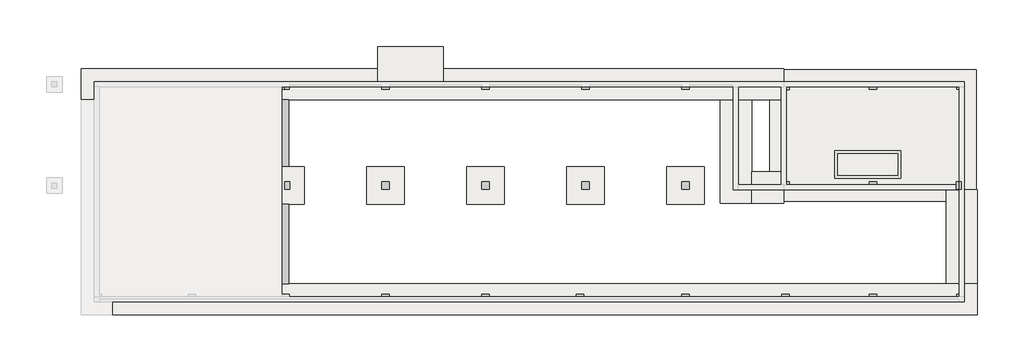
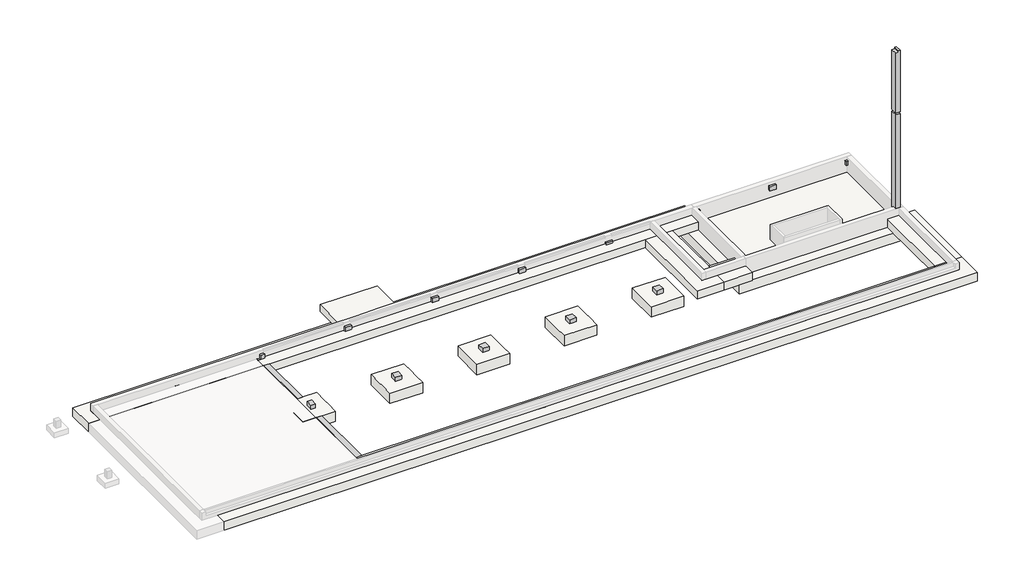
# Not in any storey, part 2 of 2: 25 columns, 8 beams, 8 slabs, 5 footings.
"""IFC4 building model written with IfcOpenShell, lengths in millimetres."""

from ifc_helpers import new_model, si_unit, frame, origin, place, context, project, spatial, polyline, outline, extrude, faceted_brep, element, save

model = new_model("IFC4")

# Units and contexts
model_context = context("Model", 3, world=origin())
ifc_project = project(units=[si_unit("LENGTHUNIT", "METRE", prefix="MILLI")], contexts=[model_context])

# Site, building
site = spatial("IfcSite", under=ifc_project)
building = spatial("IfcBuilding", under=site)

# Beams
placement = place(None, origin())
element("IfcBeam", 1, ObjectType="RC Beam_Rectangular : H_SB_AR_S16_FG_B600xH800_FG2", at=placement, inside=building, context=model_context, shape_type="Brep", body=[
    faceted_brep([(1150.0, 9199.5208589, -1350.0381366), (6000.0, 9199.5208589, -1350.0381366), (6000.0, 9199.5208589, -700.0381366), (4000.0, 9199.5208589, -700.0381366), (3500.0, 9199.5208589, -700.0381366), (1150.0, 9199.5208589, -700.0381366), (1150.0, 9799.5208589, -1350.0381366), (6000.0, 9799.5208589, -1350.0381366), (1150.0, 9799.5208589, -700.0381366), (3500.0, 9799.5208589, -700.0381366), (4000.0, 9799.5208589, -700.0381366), (6000.0, 9799.5208589, -700.0381366)], [[[0, 1, 2, 3, 4, 5]], [[0, 6, 7, 1]], [[7, 6, 8, 9, 10, 11]], [[6, 0, 5, 8]], [[1, 7, 11, 2]], [[5, 4, 3, 2, 11, 10, 9, 8]]]),
])
element("IfcBeam", 2, ObjectType="RC Beam_Rectangular : H_SB_AR_S16_FG_B600xH800_FG2", at=placement, inside=building, context=model_context, shape_type="Brep", body=[
    faceted_brep([(9000.0, 9199.5208589, -1350.0381366), (13500.0, 9199.5208589, -1350.0381366), (13500.0, 9199.5208589, -700.0381366), (11500.0, 9199.5208589, -700.0381366), (11000.0, 9199.5208589, -700.0381366), (9000.0, 9199.5208589, -700.0381366), (9000.0, 9799.5208589, -1350.0381366), (13500.0, 9799.5208589, -1350.0381366), (9000.0, 9799.5208589, -700.0381366), (11000.0, 9799.5208589, -700.0381366), (11500.0, 9799.5208589, -700.0381366), (13500.0, 9799.5208589, -700.0381366)], [[[0, 1, 2, 3, 4, 5]], [[0, 6, 7, 1]], [[7, 6, 8, 9, 10, 11]], [[6, 0, 5, 8]], [[1, 7, 11, 2]], [[5, 4, 3, 2, 11, 10, 9, 8]]]),
])
element("IfcBeam", 3, ObjectType="RC Beam_Rectangular : H_SB_AR_S16_FG_B500xH700_FB1", at=placement, inside=building, context=model_context, shape_type="SweptSolid", body=[
    extrude(outline(polyline([(4000.0, 9799.5208589), (3500.0, 9799.5208589), (3500.0, 16349.5208589), (4000.0, 16349.5208589), (4000.0, 9799.5208589)])), frame((0.0, 0.0, -1250.0381366), z_axis=(0.0, 0.0, 1.0), x_axis=(1.0, 0.0, 0.0)), (0.0, 0.0, 1.0), 550.0),
])
element("IfcBeam", 4, ObjectType="RC Beam_Rectangular : H_SB_AR_S16_FG_B500xH700_FB1", at=placement, inside=building, context=model_context, shape_type="SweptSolid", body=[
    extrude(outline(polyline([(11500.0, 9799.5208589), (11000.0, 9799.5208589), (11000.0, 16349.5208589), (11500.0, 16349.5208589), (11500.0, 9799.5208589)])), frame((0.0, 0.0, -1250.0381366), z_axis=(0.0, 0.0, 1.0), x_axis=(1.0, 0.0, 0.0)), (0.0, 0.0, 1.0), 550.0),
])
element("IfcBeam", 5, ObjectType="RC Beam_Rectangular : H_SB_AR_S16_FG_B500xH700_FB1", at=placement, inside=building, context=model_context, shape_type="SweptSolid", body=[
    extrude(outline(polyline([(11500.0, 1649.5208589), (11000.0, 1649.5208589), (11000.0, 9199.5208589), (11500.0, 9199.5208589), (11500.0, 1649.5208589)])), frame((0.0, 0.0, -1250.0381366), z_axis=(0.0, 0.0, 1.0), x_axis=(1.0, 0.0, 0.0)), (0.0, 0.0, 1.0), 550.0),
])
element("IfcBeam", 6, ObjectType="RC Beam_Rectangular : H_SB_AR_S16_FG_B500xH700_FG1", at=placement, inside=building, context=model_context, shape_type="SweptSolid", body=[
    extrude(outline(polyline([(7250.0, 16349.5208589), (7750.0, 16349.5208589), (7750.0, 10999.5208589), (7250.0, 10999.5208589), (7250.0, 16349.5208589)])), frame((0.0, 0.0, -1250.0381366), z_axis=(0.0, 0.0, 1.0), x_axis=(1.0, 0.0, 0.0)), (0.0, 0.0, 1.0), 550.0),
])
element("IfcBeam", 7, ObjectType="RC Beam_Rectangular : H_SB_AR_S16_FG_B500xH700_FG1", at=placement, inside=building, context=model_context, shape_type="SweptSolid", body=[
    extrude(outline(polyline([(14750.0, 16349.5208589), (15250.0, 16349.5208589), (15250.0, 10999.5208589), (14750.0, 10999.5208589), (14750.0, 16349.5208589)])), frame((0.0, 0.0, -1250.0381366), z_axis=(0.0, 0.0, 1.0), x_axis=(1.0, 0.0, 0.0)), (0.0, 0.0, 1.0), 700.0),
])
element("IfcBeam", 8, ObjectType="RC Beam_Rectangular : H_SB_AR_S16_FG_B500xH700_FG1", at=placement, inside=building, context=model_context, shape_type="SweptSolid", body=[
    extrude(outline(polyline([(15250.0, 1649.5208589), (14750.0, 1649.5208589), (14750.0, 7999.5208589), (15250.0, 7999.5208589), (15250.0, 1649.5208589)])), frame((0.0, 0.0, -1250.0381366), z_axis=(0.0, 0.0, 1.0), x_axis=(1.0, 0.0, 0.0)), (0.0, 0.0, 1.0), 700.0),
])

# Columns
element("IfcColumn", 9, ObjectType="RC_Column_Rectangular : H_SC_AR_S15_UG_W600xL600_C2", at=placement, inside=building, context=model_context, shape_type="Brep", body=[
    faceted_brep([(300.0, 17799.5208589, -850.0381366), (300.0, 17199.5208589, -850.0381366), (-300.0, 17199.5208589, -850.0381366), (-300.0, 17799.5208589, -850.0381366), (300.0, 17799.5208589, -550.0381366), (300.0, 17399.5208589, -550.0381366), (300.0, 17399.5208589, -700.0381366), (300.0, 17199.5208589, -700.0381366), (-300.0, 17199.5208589, -550.0381366), (-300.0, 17399.5208589, -550.0381366), (-300.0, 17799.5208589, -550.0381366), (100.0, 17199.5208589, -550.0381366), (100.0, 17399.5208589, -550.0381366), (100.0, 17399.5208589, -700.0381366), (100.0, 17199.5208589, -700.0381366)], [[[0, 1, 2, 3]], [[1, 0, 4, 5, 6, 7]], [[3, 2, 8, 9, 10]], [[0, 3, 10, 4]], [[8, 11, 12, 5, 4, 10, 9]], [[6, 13, 14, 7]], [[13, 12, 11, 14]], [[12, 13, 6, 5]], [[2, 1, 7, 14, 11, 8]]]),
])
element("IfcColumn", 10, ObjectType="RC_Column_Rectangular : H_SC_AR_S15_UG_W600xL600_C2", at=placement, inside=building, context=model_context, shape_type="SweptSolid", body=[
    extrude(outline(polyline([(17799.5208589, -850.0381366), (17199.5208589, -850.0381366), (17199.5208589, -700.0381366), (17399.5208589, -700.0381366), (17399.5208589, -550.0381366), (17799.5208589, -550.0381366), (17799.5208589, -850.0381366)])), frame((7200.0, 0.0, 0.0), z_axis=(1.0, 0.0, 0.0), x_axis=(0.0, 1.0, 0.0)), (0.0, 0.0, 1.0), 600.0),
])
element("IfcColumn", 11, ObjectType="RC_Column_Rectangular : H_SC_AR_S15_UG_W600xL600_C2", at=placement, inside=building, context=model_context, shape_type="Brep", body=[
    faceted_brep([(15300.0, 17799.5208589, -850.0381366), (15300.0, 17199.5208589, -850.0381366), (14700.0, 17199.5208589, -850.0381366), (14700.0, 17799.5208589, -850.0381366), (15300.0, 17799.5208589, -550.0381366), (15300.0, 17399.5208589, -550.0381366), (15300.0, 17399.5208589, -150.0381366), (15300.0, 17199.5208589, -150.0381366), (14950.0, 17199.5208589, -150.0381366), (14950.0, 17199.5208589, -550.0381366), (14700.0, 17199.5208589, -550.0381366), (14700.0, 17399.5208589, -550.0381366), (14700.0, 17799.5208589, -550.0381366), (14950.0, 17399.5208589, -150.0381366), (14950.0, 17399.5208589, -550.0381366)], [[[0, 1, 2, 3]], [[1, 0, 4, 5, 6, 7]], [[2, 1, 7, 8, 9, 10]], [[3, 2, 10, 11, 12]], [[0, 3, 12, 4]], [[8, 7, 6, 13]], [[14, 9, 8, 13]], [[9, 14, 5, 4, 12, 11, 10]], [[5, 14, 13, 6]]]),
])
element("IfcColumn", 12, ObjectType="RC_Column_Rectangular : H_SC_AR_S15_UG_W600xL600_C2", at=placement, inside=building, context=model_context, shape_type="SweptSolid", body=[
    extrude(outline(polyline([(17799.5208589, -850.0381366), (17199.5208589, -850.0381366), (17199.5208589, -150.0381366), (17399.5208589, -150.0381366), (17399.5208589, -550.0381366), (17799.5208589, -550.0381366), (17799.5208589, -850.0381366)])), frame((22700.0, 0.0, 0.0), z_axis=(1.0, 0.0, 0.0), x_axis=(0.0, 1.0, 0.0)), (0.0, 0.0, 1.0), 600.0),
])
element("IfcColumn", 13, ObjectType="RC_Column_Rectangular : H_SC_AR_S15_UG_W600xL600_C2", at=placement, inside=building, context=model_context, shape_type="SweptSolid", body=[
    extrude(outline(polyline([(17799.5208589, -850.0381366), (17199.5208589, -850.0381366), (17199.5208589, -150.0381366), (17399.5208589, -150.0381366), (17399.5208589, -550.0381366), (17799.5208589, -550.0381366), (17799.5208589, -850.0381366)])), frame((30700.0, 0.0, 0.0), z_axis=(1.0, 0.0, 0.0), x_axis=(0.0, 1.0, 0.0)), (0.0, 0.0, 1.0), 600.0),
])
element("IfcColumn", 14, ObjectType="RC_Column_Rectangular : H_SC_AR_S15_UG_W600xL600_C2", at=placement, inside=building, context=model_context, shape_type="SweptSolid", body=[
    extrude(outline(polyline([(17799.5208589, -850.0381366), (17199.5208589, -850.0381366), (17199.5208589, -150.0381366), (17399.5208589, -150.0381366), (17399.5208589, -550.0381366), (17799.5208589, -550.0381366), (17799.5208589, -850.0381366)])), frame((38700.0, 0.0, 0.0), z_axis=(1.0, 0.0, 0.0), x_axis=(0.0, 1.0, 0.0)), (0.0, 0.0, 1.0), 600.0),
])
element("IfcColumn", 15, ObjectType="RC_Column_Rectangular : H_SC_AR_S15_UG_W600xL600_C2", at=placement, inside=building, context=model_context, shape_type="SweptSolid", body=[
    extrude(outline(polyline([(17799.5208589, -850.0381366), (17199.5208589, -850.0381366), (17199.5208589, -359.953022), (17399.5208589, -359.953022), (17399.5208589, -550.0381366), (17799.5208589, -550.0381366), (17799.5208589, -850.0381366)])), frame((46700.0, 0.0, 0.0), z_axis=(1.0, 0.0, 0.0), x_axis=(0.0, 1.0, 0.0)), (0.0, 0.0, 1.0), 600.0),
])
element("IfcColumn", 16, ObjectType="RC_Column_Rectangular : H_SC_AR_S15_UG_W600xL600_C2", at=placement, inside=building, context=model_context, shape_type="Brep", body=[
    faceted_brep([(69300.0, 799.5208589, -850.0381366), (69300.0, 199.5208589, -850.0381366), (68700.0, 199.5208589, -850.0381366), (68700.0, 799.5208589, -850.0381366), (69300.0, 799.5208589, -550.0381366), (69300.0, 599.5208589, -550.0381366), (69300.0, 199.5208589, -550.0381366), (68700.0, 199.5208589, -550.0381366), (68700.0, 599.5208589, -550.0381366), (68700.0, 599.5208589, -150.0381366), (68700.0, 799.5208589, -150.0381366), (68900.0, 799.5208589, -150.0381366), (68900.0, 799.5208589, -550.0381366), (68900.0, 599.5208589, -150.0381366), (68900.0, 599.5208589, -550.0381366)], [[[0, 1, 2, 3]], [[1, 0, 4, 5, 6]], [[2, 1, 6, 7]], [[3, 2, 7, 8, 9, 10]], [[0, 3, 10, 11, 12, 4]], [[10, 9, 13, 11]], [[9, 8, 14, 13]], [[4, 12, 14, 8, 7, 6, 5]], [[14, 12, 11, 13]]]),
])
element("IfcColumn", 17, ObjectType="RC_Column_Rectangular : H_SC_AR_S15_UG_W600xL600_C2", at=placement, inside=building, context=model_context, shape_type="SweptSolid", body=[
    extrude(outline(polyline([(799.5208589, -850.0381366), (199.5208589, -850.0381366), (199.5208589, -550.0381366), (599.5208589, -550.0381366), (599.5208589, -150.0381366), (799.5208589, -150.0381366), (799.5208589, -850.0381366)])), frame((61700.0, 0.0, 0.0), z_axis=(1.0, 0.0, 0.0), x_axis=(0.0, 1.0, 0.0)), (0.0, 0.0, 1.0), 600.0),
])
element("IfcColumn", 18, ObjectType="RC_Column_Rectangular : H_SC_AR_S15_UG_W600xL600_C2", at=placement, inside=building, context=model_context, shape_type="SweptSolid", body=[
    extrude(outline(polyline([(799.5208589, -850.0381366), (199.5208589, -850.0381366), (199.5208589, -550.0381366), (599.5208589, -550.0381366), (599.5208589, -150.0381366), (799.5208589, -150.0381366), (799.5208589, -850.0381366)])), frame((54700.0, 0.0, 0.0), z_axis=(1.0, 0.0, 0.0), x_axis=(0.0, 1.0, 0.0)), (0.0, 0.0, 1.0), 600.0),
])
element("IfcColumn", 19, ObjectType="RC_Column_Rectangular : H_SC_AR_S15_UG_W600xL600_C2", at=placement, inside=building, context=model_context, shape_type="SweptSolid", body=[
    extrude(outline(polyline([(799.5208589, -850.0381366), (199.5208589, -850.0381366), (199.5208589, -550.0381366), (599.5208589, -550.0381366), (599.5208589, -150.0381366), (799.5208589, -150.0381366), (799.5208589, -850.0381366)])), frame((46700.0, 0.0, 0.0), z_axis=(1.0, 0.0, 0.0), x_axis=(0.0, 1.0, 0.0)), (0.0, 0.0, 1.0), 600.0),
])
element("IfcColumn", 20, ObjectType="RC_Column_Rectangular : H_SC_AR_S15_UG_W600xL600_C2", at=placement, inside=building, context=model_context, shape_type="SweptSolid", body=[
    extrude(outline(polyline([(799.5208589, -850.0381366), (199.5208589, -850.0381366), (199.5208589, -550.0381366), (599.5208589, -550.0381366), (599.5208589, -150.0381366), (799.5208589, -150.0381366), (799.5208589, -850.0381366)])), frame((38250.0, 0.0, 0.0), z_axis=(1.0, 0.0, 0.0), x_axis=(0.0, 1.0, 0.0)), (0.0, 0.0, 1.0), 600.0),
])
element("IfcColumn", 21, ObjectType="RC_Column_Rectangular : H_SC_AR_S15_UG_W600xL600_C2", at=placement, inside=building, context=model_context, shape_type="SweptSolid", body=[
    extrude(outline(polyline([(799.5208589, -850.0381366), (199.5208589, -850.0381366), (199.5208589, -550.0381366), (599.5208589, -550.0381366), (599.5208589, -150.0381366), (799.5208589, -150.0381366), (799.5208589, -850.0381366)])), frame((30700.0, 0.0, 0.0), z_axis=(1.0, 0.0, 0.0), x_axis=(0.0, 1.0, 0.0)), (0.0, 0.0, 1.0), 600.0),
])
element("IfcColumn", 22, ObjectType="RC_Column_Rectangular : H_SC_AR_S15_UG_W600xL600_C2", at=placement, inside=building, context=model_context, shape_type="SweptSolid", body=[
    extrude(outline(polyline([(799.5208589, -850.0381366), (199.5208589, -850.0381366), (199.5208589, -550.0381366), (599.5208589, -550.0381366), (599.5208589, -150.0381366), (799.5208589, -150.0381366), (799.5208589, -850.0381366)])), frame((22700.0, 0.0, 0.0), z_axis=(1.0, 0.0, 0.0), x_axis=(0.0, 1.0, 0.0)), (0.0, 0.0, 1.0), 600.0),
])
element("IfcColumn", 23, ObjectType="RC_Column_Rectangular : H_SC_AR_S15_AG_W600xL600_C2", at=placement, inside=building, context=model_context, shape_type="SweptSolid", body=[
    extrude(outline(polyline([(15350.0, 9799.5208589), (15350.0, 9199.5208589), (14950.0, 9199.5208589), (14950.0, 9799.5208589), (15350.0, 9799.5208589)])), frame((0.0, 0.0, -550.0381366), z_axis=(0.0, 0.0, 1.0), x_axis=(1.0, 0.0, 0.0)), (0.0, 0.0, 1.0), 400.0),
])
element("IfcColumn", 24, ObjectType="RC_Column_Rectangular : H_SC_AR_S15_AG_W600xL600_C2", at=placement, inside=building, context=model_context, shape_type="SweptSolid", body=[
    extrude(outline(polyline([(23300.0, 9799.5208589), (23300.0, 9199.5208589), (22700.0, 9199.5208589), (22700.0, 9799.5208589), (23300.0, 9799.5208589)])), frame((0.0, 0.0, -550.0381366), z_axis=(0.0, 0.0, 1.0), x_axis=(1.0, 0.0, 0.0)), (0.0, 0.0, 1.0), 400.0),
])
element("IfcColumn", 25, ObjectType="RC_Column_Rectangular : H_SC_AR_S15_AG_W600xL600_C2", at=placement, inside=building, context=model_context, shape_type="SweptSolid", body=[
    extrude(outline(polyline([(31300.0, 9799.5208589), (31300.0, 9199.5208589), (30700.0, 9199.5208589), (30700.0, 9799.5208589), (31300.0, 9799.5208589)])), frame((0.0, 0.0, -550.0381366), z_axis=(0.0, 0.0, 1.0), x_axis=(1.0, 0.0, 0.0)), (0.0, 0.0, 1.0), 400.0),
])
element("IfcColumn", 26, ObjectType="RC_Column_Rectangular : H_SC_AR_S15_AG_W600xL600_C2", at=placement, inside=building, context=model_context, shape_type="SweptSolid", body=[
    extrude(outline(polyline([(39300.0, 9799.5208589), (39300.0, 9199.5208589), (38700.0, 9199.5208589), (38700.0, 9799.5208589), (39300.0, 9799.5208589)])), frame((0.0, 0.0, -550.0381366), z_axis=(0.0, 0.0, 1.0), x_axis=(1.0, 0.0, 0.0)), (0.0, 0.0, 1.0), 400.0),
])
element("IfcColumn", 27, ObjectType="RC_Column_Rectangular : H_SC_AR_S15_AG_W600xL600_C2", at=placement, inside=building, context=model_context, shape_type="SweptSolid", body=[
    extrude(outline(polyline([(47300.0, 9799.5208589), (47300.0, 9199.5208589), (46700.0, 9199.5208589), (46700.0, 9799.5208589), (47300.0, 9799.5208589)])), frame((0.0, 0.0, -550.0381366), z_axis=(0.0, 0.0, 1.0), x_axis=(1.0, 0.0, 0.0)), (0.0, 0.0, 1.0), 400.0),
])
element("IfcColumn", 28, ObjectType="RC_Column_Rectangular : H_SC_AR_S15_AG_W600xL600_C2", at=placement, inside=building, context=model_context, shape_type="SweptSolid", body=[
    extrude(outline(polyline([(55300.0, 9799.5208589), (55300.0, 9549.5208589), (55050.0, 9549.5208589), (55050.0, 9799.5208589), (55300.0, 9799.5208589)])), frame((0.0, 0.0, -550.0381366), z_axis=(0.0, 0.0, 1.0), x_axis=(1.0, 0.0, 0.0)), (0.0, 0.0, 1.0), 400.0),
])
element("IfcColumn", 29, ObjectType="RC_Column_Rectangular : H_SC_AR_S15_AG_W600xL600_C2", at=placement, inside=building, context=model_context, shape_type="SweptSolid", body=[
    extrude(outline(polyline([(61700.0, 9799.5208589), (62300.0, 9799.5208589), (62300.0, 9549.5208589), (61700.0, 9549.5208589), (61700.0, 9799.5208589)])), frame((0.0, 0.0, -550.0381366), z_axis=(0.0, 0.0, 1.0), x_axis=(1.0, 0.0, 0.0)), (0.0, 0.0, 1.0), 400.0),
])
element("IfcColumn", 30, ObjectType="RC_Column_Rectangular : H_SC_AR_S15_AG_W600xL600_C2", at=placement, inside=building, context=model_context, shape_type="Brep", body=[
    faceted_brep([(68650.0, 9799.5208589, -550.0381366), (68900.0, 9799.5208589, -550.0381366), (68900.0, 9549.5208589, -550.0381366), (68650.0, 9549.5208589, -550.0381366), (68900.0, 9799.5208589, 149.9618634), (68900.0, 9549.5208589, 149.9618634), (68650.0, 9549.5208589, 149.9618634), (69050.0, 9799.5208589, 149.9618634), (69050.0, 9199.5208589, 149.9618634), (68650.0, 9199.5208589, 149.9618634), (69050.0, 9799.5208589, 9269.9618634), (69050.0, 9199.5208589, 9269.9618634), (68650.0, 9199.5208589, 9269.9618634), (68650.0, 9799.5208589, 9269.9618634)], [[[0, 1, 2, 3]], [[1, 4, 5, 2]], [[6, 5, 4, 7, 8, 9]], [[5, 6, 3, 2]], [[8, 7, 10, 11]], [[12, 11, 10, 13]], [[9, 8, 11, 12]], [[0, 3, 6, 9, 12, 13]], [[1, 0, 13, 10, 7, 4]]]),
    faceted_brep([(69050.0, 9199.5208589, 9449.9618634), (69050.0, 9199.5208589, 15409.9618634), (68900.0, 9199.5208589, 15409.9618634), (68900.0, 9199.5208589, 15259.9618634), (68650.0, 9199.5208589, 15259.9618634), (68650.0, 9199.5208589, 9449.9618634), (68650.0, 9799.5208589, 9449.9618634), (68650.0, 9799.5208589, 15259.9618634), (69050.0, 9799.5208589, 15409.9618634), (69050.0, 9799.5208589, 9449.9618634), (68900.0, 9799.5208589, 15259.9618634), (68900.0, 9799.5208589, 15409.9618634)], [[[0, 1, 2, 3, 4, 5]], [[6, 5, 4, 7]], [[8, 9, 6, 7, 10, 11]], [[1, 8, 11, 2]], [[0, 5, 6, 9]], [[8, 1, 0, 9]], [[3, 10, 7, 4]], [[10, 3, 2, 11]]]),
])
element("IfcColumn", 31, ObjectType="RC_Column_Rectangular : H_SC_AR_S15_UG_W600xL600_C2", at=placement, inside=building, context=model_context, shape_type="SweptSolid", body=[
    extrude(outline(polyline([(68700.0, 17199.5208589), (68700.0, 17399.5208589), (68900.0, 17399.5208589), (68900.0, 17199.5208589), (68700.0, 17199.5208589)])), frame((0.0, 0.0, -550.0381366), z_axis=(0.0, 0.0, 1.0), x_axis=(1.0, 0.0, 0.0)), (0.0, 0.0, 1.0), 400.0),
])
element("IfcColumn", 32, ObjectType="RC_Column_Rectangular : H_SC_AR_S15_UG_W600xL600_C2", at=placement, inside=building, context=model_context, shape_type="SweptSolid", body=[
    extrude(outline(polyline([(62300.0, 17199.5208589), (61700.0, 17199.5208589), (61700.0, 17399.5208589), (62300.0, 17399.5208589), (62300.0, 17199.5208589)])), frame((0.0, 0.0, -550.0381366), z_axis=(0.0, 0.0, 1.0), x_axis=(1.0, 0.0, 0.0)), (0.0, 0.0, 1.0), 400.0),
])
element("IfcColumn", 33, ObjectType="RC_Column_Rectangular : H_SC_AR_S15_AG_W600xL600_C2", at=placement, inside=building, context=model_context, shape_type="SweptSolid", body=[
    extrude(outline(polyline([(54850.0, 17749.5208589), (54850.0, 17399.5208589), (54700.0, 17399.5208589), (54700.0, 17749.5208589), (54850.0, 17749.5208589)])), frame((0.0, 0.0, -550.0381366), z_axis=(0.0, 0.0, 1.0), x_axis=(1.0, 0.0, 0.0)), (0.0, 0.0, 1.0), 400.0),
    extrude(outline(polyline([(55300.0, 17399.5208589), (55300.0, 17149.5208589), (55050.0, 17149.5208589), (55050.0, 17399.5208589), (55300.0, 17399.5208589)])), frame((0.0, 0.0, -550.0381366), z_axis=(0.0, 0.0, 1.0), x_axis=(1.0, 0.0, 0.0)), (0.0, 0.0, 1.0), 400.0),
])

# Footings
element("IfcFooting", 34, ObjectType="H_SF_AR_B01_Wall FDN_T800", at=placement, inside=building, context=model_context, shape_type="Brep", body=[
    faceted_brep([(54850.0, 18849.5208589, -550.0381366), (54850.0, 16349.5208589, -550.0381366), (54850.0, 16349.5208589, -1350.0381366), (54850.0, 18849.5208589, -1350.0381366), (-1350.0, 16349.5208589, -550.0381366), (1150.0, 16349.5208589, -550.0381366), (14750.0, 16349.5208589, -550.0381366), (15250.0, 16349.5208589, -550.0381366), (49775.0, 16349.5208589, -550.0381366), (52275.0, 16349.5208589, -550.0381366), (-1350.0, 18849.5208589, -550.0381366), (-1350.0, 18849.5208589, -1350.0381366), (-1350.0, 16349.5208589, -1350.0381366), (52275.0, 16349.5208589, -1350.0381366), (49775.0, 16349.5208589, -1350.0381366), (1150.0, 16349.5208589, -1350.0381366)], [[[0, 1, 2, 3]], [[4, 5, 6, 7, 8, 9, 1, 0, 10]], [[11, 10, 0, 3]], [[12, 11, 3, 2, 13, 14, 15]], [[4, 12, 15, 14, 13, 2, 1, 9, 8, 7, 6, 5]], [[4, 10, 11, 12]]]),
])
element("IfcFooting", 35, ObjectType="H_SF_AR_B01_Wall FDN_T800", at=placement, inside=building, context=model_context, shape_type="Brep", body=[
    faceted_brep([(70350.0, -850.4791411, -550.0381366), (70350.0, 1649.5208589, -550.0381366), (67850.0, 1649.5208589, -550.0381366), (15250.0, 1649.5208589, -550.0381366), (14750.0, 1649.5208589, -550.0381366), (1150.0, 1649.5208589, -550.0381366), (1150.0, -850.4791411, -550.0381366), (70350.0, -850.4791411, -1350.0381366), (1150.0, -850.4791411, -1350.0381366), (70350.0, 1649.5208589, -1350.0381366), (1150.0, 1649.5208589, -1350.0381366), (67850.0, 1649.5208589, -1350.0381366)], [[[0, 1, 2, 3, 4, 5, 6]], [[7, 0, 6, 8]], [[9, 7, 8, 10, 11]], [[1, 9, 11, 10, 5, 4, 3, 2]], [[1, 0, 7, 9]], [[6, 5, 10, 8]]]),
])
element("IfcFooting", 36, ObjectType="H_SF_AR_B01_Wall FDN_T800", at=placement, inside=building, context=model_context, shape_type="SweptSolid", body=[
    extrude(outline(polyline([(67850.0, 9149.5208589), (70350.0, 9149.5208589), (70350.0, 1649.5208589), (67850.0, 1649.5208589), (67850.0, 9149.5208589)])), frame((0.0, 0.0, -1350.0381366), z_axis=(0.0, 0.0, 1.0), x_axis=(1.0, 0.0, 0.0)), (0.0, 0.0, 1.0), 800.0),
])
element("IfcFooting", 37, ObjectType="H_SF_AR_B01_Wall FDN_T800", at=placement, inside=building, context=model_context, shape_type="Brep", body=[
    faceted_brep([(49775.0, 16349.5208589, -550.0381366), (49775.0, 9799.5208589, -550.0381366), (49775.0, 9199.5208589, -550.0381366), (49775.0, 8099.5208589, -550.0381366), (52275.0, 8099.5208589, -550.0381366), (52275.0, 10599.5208589, -550.0381366), (52275.0, 16349.5208589, -550.0381366), (52275.0, 16349.5208589, -1350.0381366), (52275.0, 8099.5208589, -1350.0381366), (52275.0, 10599.5208589, -1350.0381366), (49775.0, 16349.5208589, -1350.0381366), (49775.0, 8099.5208589, -1350.0381366)], [[[0, 1, 2, 3, 4, 5, 6]], [[7, 6, 5, 4, 8, 9]], [[10, 7, 9, 8, 11]], [[0, 10, 11, 3, 2, 1]], [[0, 6, 7, 10]], [[4, 3, 11, 8]]]),
])
element("IfcFooting", 38, ObjectType="H_SF_AR_B01_Wall FDN_T800", at=placement, inside=building, context=model_context, shape_type="SweptSolid", body=[
    extrude(outline(polyline([(54850.0, 10599.5208589), (54850.0, 8099.5208589), (52275.0, 8099.5208589), (52275.0, 10599.5208589), (54850.0, 10599.5208589)])), frame((0.0, 0.0, -1350.0381366), z_axis=(0.0, 0.0, 1.0), x_axis=(1.0, 0.0, 0.0)), (0.0, 0.0, 1.0), 800.0),
])

# Slabs
element("IfcSlab", 39, ObjectType="H_SF_AR_B01_MAT_Bitumen_MF1", at=placement, inside=building, context=model_context, shape_type="SweptSolid", body=[
    extrude(outline(polyline([(70250.0, 18749.5208589), (70250.0, 8249.5208589), (53750.0, 8249.5208589), (53750.0, 18749.5208589), (70250.0, 18749.5208589)])), frame((0.0, 0.0, -2350.0381366), z_axis=(0.0, 0.0, 1.0), x_axis=(1.0, 0.0, 0.0)), (0.0, 0.0, 1.0), 1000.0),
])
element("IfcSlab", 40, ObjectType="H_SF_AR_B01_MAT_Bitumen_MF2", at=placement, inside=building, context=model_context, shape_type="Brep", body=[
    faceted_brep([(27625.0, 20624.5208589, -550.0381366), (27625.0, 17799.5208589, -550.0381366), (22375.0, 17799.5208589, -550.0381366), (22375.0, 20624.5208589, -550.0381366), (27625.0, 20624.5208589, 99.9618634), (22375.0, 20624.5208589, 99.9618634), (22375.0, 17799.5208589, 99.9618634), (27625.0, 17799.5208589, 99.9618634), (22375.0, 17799.5208589, -50.0381366)], [[[0, 1, 2, 3]], [[4, 5, 6, 7]], [[1, 0, 4, 7]], [[2, 1, 7, 6, 8]], [[3, 2, 8, 6, 5]], [[0, 3, 5, 4]]]),
])
element("IfcSlab", 41, ObjectType="Foundation Rectangular (Non-Pile) : H_SF_AR_S18_W2500xL2500xT1000_Bitumen_F1", at=placement, inside=building, context=model_context, shape_type="Brep", body=[
    faceted_brep([(9000.0, 10999.5208589, -1550.0381366), (9000.0, 7999.5208589, -1550.0381366), (6000.0, 7999.5208589, -1550.0381366), (6000.0, 10999.5208589, -1550.0381366), (6000.0, 10999.5208589, -700.0381366), (7250.0, 10999.5208589, -700.0381366), (7750.0, 10999.5208589, -700.0381366), (9000.0, 10999.5208589, -700.0381366), (6000.0, 7999.5208589, -700.0381366), (6000.0, 9199.5208589, -700.0381366), (6000.0, 9799.5208589, -700.0381366), (9000.0, 7999.5208589, -700.0381366), (7750.0, 7999.5208589, -700.0381366), (7250.0, 7999.5208589, -700.0381366), (9000.0, 9799.5208589, -700.0381366), (9000.0, 9199.5208589, -700.0381366)], [[[0, 1, 2, 3]], [[0, 3, 4, 5, 6, 7]], [[3, 2, 8, 9, 10, 4]], [[2, 1, 11, 12, 13, 8]], [[1, 0, 7, 14, 15, 11]], [[7, 6, 5, 4, 10, 9, 8, 13, 12, 11, 15, 14]]]),
])
element("IfcSlab", 42, ObjectType="Foundation Rectangular (Non-Pile) : H_SF_AR_S18_W2500xL2500xT1000_Bitumen_F1", at=placement, inside=building, context=model_context, shape_type="Brep", body=[
    faceted_brep([(16500.0, 10999.5208589, -550.0381366), (15250.0, 10999.5208589, -550.0381366), (14750.0, 10999.5208589, -550.0381366), (13500.0, 10999.5208589, -550.0381366), (13500.0, 7999.5208589, -550.0381366), (14750.0, 7999.5208589, -550.0381366), (15250.0, 7999.5208589, -550.0381366), (16500.0, 7999.5208589, -550.0381366), (16500.0, 9149.5208589, -550.0381366), (16500.0, 9749.5208589, -550.0381366), (16500.0, 10999.5208589, -1550.0381366), (16500.0, 7999.5208589, -1550.0381366), (13500.0, 7999.5208589, -1550.0381366), (13500.0, 10999.5208589, -1550.0381366)], [[[0, 1, 2, 3, 4, 5, 6, 7, 8, 9]], [[10, 11, 12, 13]], [[3, 2, 1, 0, 10, 13]], [[4, 3, 13, 12]], [[7, 6, 5, 4, 12, 11]], [[0, 9, 8, 7, 11, 10]]]),
])
element("IfcSlab", 43, ObjectType="Foundation Rectangular (Non-Pile) : H_SF_AR_S18_W2500xL2500xT1000_Bitumen_F1", at=placement, inside=building, context=model_context, shape_type="Brep", body=[
    faceted_brep([(24500.0, 10999.5208589, -550.0381366), (21500.0, 10999.5208589, -550.0381366), (21500.0, 9749.5208589, -550.0381366), (21500.0, 9149.5208589, -550.0381366), (21500.0, 7999.5208589, -550.0381366), (24500.0, 7999.5208589, -550.0381366), (24500.0, 9149.5208589, -550.0381366), (24500.0, 9749.5208589, -550.0381366), (24500.0, 10999.5208589, -1550.0381366), (24500.0, 7999.5208589, -1550.0381366), (21500.0, 7999.5208589, -1550.0381366), (21500.0, 10999.5208589, -1550.0381366)], [[[0, 1, 2, 3, 4, 5, 6, 7]], [[8, 9, 10, 11]], [[1, 0, 8, 11]], [[4, 3, 2, 1, 11, 10]], [[5, 4, 10, 9]], [[0, 7, 6, 5, 9, 8]]]),
])
element("IfcSlab", 44, ObjectType="Foundation Rectangular (Non-Pile) : H_SF_AR_S18_W2500xL2500xT1000_Bitumen_F1", at=placement, inside=building, context=model_context, shape_type="Brep", body=[
    faceted_brep([(32500.0, 10999.5208589, -550.0381366), (29500.0, 10999.5208589, -550.0381366), (29500.0, 9749.5208589, -550.0381366), (29500.0, 9149.5208589, -550.0381366), (29500.0, 7999.5208589, -550.0381366), (32500.0, 7999.5208589, -550.0381366), (32500.0, 9149.5208589, -550.0381366), (32500.0, 9749.5208589, -550.0381366), (32500.0, 10999.5208589, -1550.0381366), (32500.0, 7999.5208589, -1550.0381366), (29500.0, 7999.5208589, -1550.0381366), (29500.0, 10999.5208589, -1550.0381366)], [[[0, 1, 2, 3, 4, 5, 6, 7]], [[8, 9, 10, 11]], [[1, 0, 8, 11]], [[4, 3, 2, 1, 11, 10]], [[5, 4, 10, 9]], [[0, 7, 6, 5, 9, 8]]]),
])
element("IfcSlab", 45, ObjectType="Foundation Rectangular (Non-Pile) : H_SF_AR_S18_W2500xL2500xT1000_Bitumen_F1", at=placement, inside=building, context=model_context, shape_type="Brep", body=[
    faceted_brep([(40500.0, 10999.5208589, -550.0381366), (37500.0, 10999.5208589, -550.0381366), (37500.0, 9749.5208589, -550.0381366), (37500.0, 9149.5208589, -550.0381366), (37500.0, 7999.5208589, -550.0381366), (40500.0, 7999.5208589, -550.0381366), (40500.0, 9149.5208589, -550.0381366), (40500.0, 9749.5208589, -550.0381366), (40500.0, 10999.5208589, -1550.0381366), (40500.0, 7999.5208589, -1550.0381366), (37500.0, 7999.5208589, -1550.0381366), (37500.0, 10999.5208589, -1550.0381366)], [[[0, 1, 2, 3, 4, 5, 6, 7]], [[8, 9, 10, 11]], [[1, 0, 8, 11]], [[4, 3, 2, 1, 11, 10]], [[5, 4, 10, 9]], [[0, 7, 6, 5, 9, 8]]]),
])
element("IfcSlab", 46, ObjectType="Foundation Rectangular (Non-Pile) : H_SF_AR_S18_W2500xL2500xT1000_Bitumen_F1", at=placement, inside=building, context=model_context, shape_type="Brep", body=[
    faceted_brep([(48500.0, 10999.5208589, -550.0381366), (45500.0, 10999.5208589, -550.0381366), (45500.0, 9749.5208589, -550.0381366), (45500.0, 9149.5208589, -550.0381366), (45500.0, 7999.5208589, -550.0381366), (48500.0, 7999.5208589, -550.0381366), (48500.0, 9199.5208589, -550.0381366), (48500.0, 9799.5208589, -550.0381366), (48500.0, 10999.5208589, -1550.0381366), (48500.0, 7999.5208589, -1550.0381366), (45500.0, 7999.5208589, -1550.0381366), (45500.0, 10999.5208589, -1550.0381366)], [[[0, 1, 2, 3, 4, 5, 6, 7]], [[8, 9, 10, 11]], [[1, 0, 8, 11]], [[4, 3, 2, 1, 11, 10]], [[5, 4, 10, 9]], [[0, 7, 6, 5, 9, 8]]]),
])

save(model, "model.ifc")

# Revit data of these elements
# Type "RC Beam_Rectangular : H_SB_AR_S16_FG_B600xH800_FG2"
#   Type Comments = "CV-UG"
#   Type Mark = "FG2"
#   H_Q'ty Cal Type Tag = "SB-Q1A"
#   H_WM Code_1 = "A03AF032-00022 |  | M3 | Concrete Work | Superstructure Work | Structural Concrete | Cement Type-1 | 25MPa ≤ F'c (Cylinder Strength) < 30MPa |  |  |  |  | A03AF032-00022 Concrete Work Superstructure Work Structural Concrete  Cement Type-1 25MPa ≤ F'c (Cylinder Strength) < 30MPa      |  F'c (Cylinder Strength) = 24MPa"
#   H_WM Code_2 = "A03AD037-00002 |  | TON | Concrete Work | Substructure Work | Rebar Work | Deformed Bar (Non-Coat.) | 400MPa<Fy≤470MPa |  |  |  |  | A03AD037-00002 Concrete Work Substructure Work Rebar Work Deformed Bar (Non-Coat.)  400MPa<Fy≤470MPa      | ASTM A615 GRADE 60 (Fy=420MPa)"
#   H_WM Code_3 = "A03AD035-00001 |  | M2 | Concrete Work | Substructure Work | Form Work (3 times in use) | Flat Form | Dressed Lumber, Plywood or Steel Form(Wood Planks are not Allowed) incl. Chamfer |  |  |  | A03AD035-00001 Concrete Work Substructure Work Form Work (3 times in use) Flat Form     Dressed Lumber, Plywood or Steel Form(Wood Planks are not Allowed) incl. Chamfer   | Dressed Lumber, Plywood or Steel Form(Wood Planks are not Allowed) incl. Chamfer"
#   H_WM Code_4 = "A03AH056-00001 |  | M2 | Concrete Work | Concrete Protective Coating (U/G) | Bitumen/Bituminous/Asphalt Coating |  |  | A03AH056-00001 Concrete Work Concrete Protective Coating (U/G) Bitumen/Bituminous/Asphalt Coating         | Bitumen/Bituminous/Asphalt Coating"
#   H_WM Code_5 = "A03AD047-00004 |  | M2 | Concrete Work | Substructure Work | Insulation under Ground Floor | Extruded Polystyrene Insulation Board |  | 100mm≤THK | THK=(  )mm |  | A03AD047-00004 Concrete Work Substructure Work Insulation under Ground Floor Extruded Polystyrene Insulation Board       100mm≤THK | Bitumen/Bituminous/Asphalt Coating"
#   H_WM Code_6 = "A01ZZ001-00012 |  | M3 | Earth Work | - | Excavation | Soil, Mech. |  | Manual Excavation Above GWL |  |  |  | A01ZZ001-00012 Earth Work - Excavation Soil, Mech.      Manual Excavation Above GWL  | Above GWL"
#   H_WM Code_7 = "A01ZZ001-00013 |  | M3 | Earth Work | - | Excavation | Soil, Mech. |  | Manual Excavation Below GWL |  |  |  | A01ZZ001-00013 Earth Work - Excavation Soil, Mech.      Manual Excavation Below GWL  | Below GWL"
#   H_WM Code_8 = "A01ZZ003-00001 |  | M3 | Earth Work | - | Backfill | Re-use, Soil |  |  |  | Compaction=(  )% |  | A01ZZ003-00001 Earth Work - Backfill Re-use, Soil        | Compaction=( 95 )%"
#   H_WM Code_9 = "A01ZZ004-00001 |  | M3 | Earth Work | - | Disposal | Soil |  |  |  | Disposal Distance=Appx. (  )km from Site |  | A01ZZ004-00001 Earth Work - Disposal Soil        | Disposal Distance=Appx. (20 )km from Site"
#   H_WM Code_10 = "A03AH056-00001 |  | M2 | Concrete Work | Concrete Protective Coating (U/G) | Bitumen/Bituminous/Asphalt Coating |  |  | A03AH056-00001 Concrete Work Concrete Protective Coating (U/G) Bitumen/Bituminous/Asphalt Coating         | *기초바닥 Protection 은 Lean에 적용"
#   중앙부 하부근 = ""
#   중앙부 상부근 = ""
#   중앙부 보조근 = ""
#   중앙부 늑근 = ""
#   외단부 하부근 = ""
#   외단부 상부근 = ""
#   외단부 보조근 = ""
#   외단부 늑근 = ""
#   부호 = "TG2"
#   내단부 하부근 = ""
#   내단부 상부근 = ""
#   내단부 보조근 = ""
#   내단부 늑근 = ""
#   ALL 하부근 = "3-D20"
#   ALL 상부근 = "4-D20"
#   ALL 보조근 = ""
#   ALL 늑근 = "2-D10 @120"
#   H_Rebar ratio = 0.14
#   Width = 600 mm
#   Height = 800 mm
#   Length [instance default] = 1524 mm
#   b = 600 mm
#   h = 800 mm
#   hec_material3 [instance default] = none
#   hec_material2 [instance default] = none
#   hec_material1 [instance default] = none
#   Structural Material [instance default] = none
#   Assembly Code = ""
# Type "RC Beam_Rectangular : H_SB_AR_S16_FG_B500xH700_FB1"
#   Type Comments = "CV-UG"
#   Type Mark = "FB1"
#   H_Q'ty Cal Type Tag = "SB-Q1A"
#   H_WM Code_1 = "A03AF032-00022 |  | M3 | Concrete Work | Superstructure Work | Structural Concrete | Cement Type-1 | 25MPa ≤ F'c (Cylinder Strength) < 30MPa |  |  |  |  | A03AF032-00022 Concrete Work Superstructure Work Structural Concrete  Cement Type-1 25MPa ≤ F'c (Cylinder Strength) < 30MPa      |  F'c (Cylinder Strength) = 24MPa"
#   H_WM Code_2 = "A03AD037-00002 |  | TON | Concrete Work | Substructure Work | Rebar Work | Deformed Bar (Non-Coat.) | 400MPa<Fy≤470MPa |  |  |  |  | A03AD037-00002 Concrete Work Substructure Work Rebar Work Deformed Bar (Non-Coat.)  400MPa<Fy≤470MPa      | ASTM A615 GRADE 60 (Fy=420MPa)"
#   H_WM Code_3 = "A03AD035-00001 |  | M2 | Concrete Work | Substructure Work | Form Work (3 times in use) | Flat Form | Dressed Lumber, Plywood or Steel Form(Wood Planks are not Allowed) incl. Chamfer |  |  |  | A03AD035-00001 Concrete Work Substructure Work Form Work (3 times in use) Flat Form     Dressed Lumber, Plywood or Steel Form(Wood Planks are not Allowed) incl. Chamfer   | Dressed Lumber, Plywood or Steel Form(Wood Planks are not Allowed) incl. Chamfer"
#   H_WM Code_4 = "A03AH056-00001 |  | M2 | Concrete Work | Concrete Protective Coating (U/G) | Bitumen/Bituminous/Asphalt Coating |  |  | A03AH056-00001 Concrete Work Concrete Protective Coating (U/G) Bitumen/Bituminous/Asphalt Coating         | Bitumen/Bituminous/Asphalt Coating"
#   H_WM Code_5 = "A03AD047-00004 |  | M2 | Concrete Work | Substructure Work | Insulation under Ground Floor | Extruded Polystyrene Insulation Board |  | 100mm≤THK | THK=(  )mm |  | A03AD047-00004 Concrete Work Substructure Work Insulation under Ground Floor Extruded Polystyrene Insulation Board       100mm≤THK | Bitumen/Bituminous/Asphalt Coating"
#   H_WM Code_6 = "A01ZZ001-00012 |  | M3 | Earth Work | - | Excavation | Soil, Mech. |  | Manual Excavation Above GWL |  |  |  | A01ZZ001-00012 Earth Work - Excavation Soil, Mech.      Manual Excavation Above GWL  | Above GWL"
#   H_WM Code_7 = "A01ZZ001-00013 |  | M3 | Earth Work | - | Excavation | Soil, Mech. |  | Manual Excavation Below GWL |  |  |  | A01ZZ001-00013 Earth Work - Excavation Soil, Mech.      Manual Excavation Below GWL  | Below GWL"
#   H_WM Code_8 = "A01ZZ003-00001 |  | M3 | Earth Work | - | Backfill | Re-use, Soil |  |  |  | Compaction=(  )% |  | A01ZZ003-00001 Earth Work - Backfill Re-use, Soil        | Compaction=( 95 )%"
#   H_WM Code_9 = "A01ZZ004-00001 |  | M3 | Earth Work | - | Disposal | Soil |  |  |  | Disposal Distance=Appx. (  )km from Site |  | A01ZZ004-00001 Earth Work - Disposal Soil        | Disposal Distance=Appx. (20 )km from Site"
#   H_WM Code_10 = "A03AH056-00001 |  | M2 | Concrete Work | Concrete Protective Coating (U/G) | Bitumen/Bituminous/Asphalt Coating |  |  | A03AH056-00001 Concrete Work Concrete Protective Coating (U/G) Bitumen/Bituminous/Asphalt Coating         | *기초바닥 Protection 은 Lean에 적용"
#   중앙부 하부근 = ""
#   중앙부 상부근 = ""
#   중앙부 보조근 = ""
#   중앙부 늑근 = ""
#   외단부 하부근 = ""
#   외단부 상부근 = ""
#   외단부 보조근 = ""
#   외단부 늑근 = ""
#   부호 = "TG2"
#   내단부 하부근 = ""
#   내단부 상부근 = ""
#   내단부 보조근 = ""
#   내단부 늑근 = ""
#   ALL 하부근 = "3-D20"
#   ALL 상부근 = "4-D20"
#   ALL 보조근 = ""
#   ALL 늑근 = "2-D10 @120"
#   H_Rebar ratio = 0.14
#   Width = 500 mm
#   Height = 700 mm
#   Length [instance default] = 1524 mm
#   b = 500 mm
#   h = 700 mm
#   hec_material3 [instance default] = none
#   hec_material2 [instance default] = none
#   hec_material1 [instance default] = none
#   Structural Material [instance default] = none
#   Assembly Code = ""
# Type "RC Beam_Rectangular : H_SB_AR_S16_FG_B500xH700_FG1"
#   Type Comments = "CV-UG"
#   Type Mark = "FG1"
#   H_Q'ty Cal Type Tag = "SB-Q1A"
#   H_WM Code_1 = "A03AF032-00022 |  | M3 | Concrete Work | Superstructure Work | Structural Concrete | Cement Type-1 | 25MPa ≤ F'c (Cylinder Strength) < 30MPa |  |  |  |  | A03AF032-00022 Concrete Work Superstructure Work Structural Concrete  Cement Type-1 25MPa ≤ F'c (Cylinder Strength) < 30MPa      |  F'c (Cylinder Strength) = 24MPa"
#   H_WM Code_2 = "A03AD037-00002 |  | TON | Concrete Work | Substructure Work | Rebar Work | Deformed Bar (Non-Coat.) | 400MPa<Fy≤470MPa |  |  |  |  | A03AD037-00002 Concrete Work Substructure Work Rebar Work Deformed Bar (Non-Coat.)  400MPa<Fy≤470MPa      | ASTM A615 GRADE 60 (Fy=420MPa)"
#   H_WM Code_3 = "A03AD035-00001 |  | M2 | Concrete Work | Substructure Work | Form Work (3 times in use) | Flat Form | Dressed Lumber, Plywood or Steel Form(Wood Planks are not Allowed) incl. Chamfer |  |  |  | A03AD035-00001 Concrete Work Substructure Work Form Work (3 times in use) Flat Form     Dressed Lumber, Plywood or Steel Form(Wood Planks are not Allowed) incl. Chamfer   | Dressed Lumber, Plywood or Steel Form(Wood Planks are not Allowed) incl. Chamfer"
#   H_WM Code_4 = "A03AH056-00001 |  | M2 | Concrete Work | Concrete Protective Coating (U/G) | Bitumen/Bituminous/Asphalt Coating |  |  | A03AH056-00001 Concrete Work Concrete Protective Coating (U/G) Bitumen/Bituminous/Asphalt Coating         | Bitumen/Bituminous/Asphalt Coating"
#   H_WM Code_5 = "A03AD047-00004 |  | M2 | Concrete Work | Substructure Work | Insulation under Ground Floor | Extruded Polystyrene Insulation Board |  | 100mm≤THK | THK=(  )mm |  | A03AD047-00004 Concrete Work Substructure Work Insulation under Ground Floor Extruded Polystyrene Insulation Board       100mm≤THK | Bitumen/Bituminous/Asphalt Coating"
#   H_WM Code_6 = "A01ZZ001-00012 |  | M3 | Earth Work | - | Excavation | Soil, Mech. |  | Manual Excavation Above GWL |  |  |  | A01ZZ001-00012 Earth Work - Excavation Soil, Mech.      Manual Excavation Above GWL  | Above GWL"
#   H_WM Code_7 = "A01ZZ001-00013 |  | M3 | Earth Work | - | Excavation | Soil, Mech. |  | Manual Excavation Below GWL |  |  |  | A01ZZ001-00013 Earth Work - Excavation Soil, Mech.      Manual Excavation Below GWL  | Below GWL"
#   H_WM Code_8 = "A01ZZ003-00001 |  | M3 | Earth Work | - | Backfill | Re-use, Soil |  |  |  | Compaction=(  )% |  | A01ZZ003-00001 Earth Work - Backfill Re-use, Soil        | Compaction=( 95 )%"
#   H_WM Code_9 = "A01ZZ004-00001 |  | M3 | Earth Work | - | Disposal | Soil |  |  |  | Disposal Distance=Appx. (  )km from Site |  | A01ZZ004-00001 Earth Work - Disposal Soil        | Disposal Distance=Appx. (20 )km from Site"
#   H_WM Code_10 = "A03AH056-00001 |  | M2 | Concrete Work | Concrete Protective Coating (U/G) | Bitumen/Bituminous/Asphalt Coating |  |  | A03AH056-00001 Concrete Work Concrete Protective Coating (U/G) Bitumen/Bituminous/Asphalt Coating         | *기초바닥 Protection 은 Lean에 적용"
#   중앙부 하부근 = ""
#   중앙부 상부근 = ""
#   중앙부 보조근 = ""
#   중앙부 늑근 = ""
#   외단부 하부근 = ""
#   외단부 상부근 = ""
#   외단부 보조근 = ""
#   외단부 늑근 = ""
#   부호 = "TG2"
#   내단부 하부근 = ""
#   내단부 상부근 = ""
#   내단부 보조근 = ""
#   내단부 늑근 = ""
#   ALL 하부근 = "3-D20"
#   ALL 상부근 = "4-D20"
#   ALL 보조근 = ""
#   ALL 늑근 = "2-D10 @120"
#   H_Rebar ratio = 0.14
#   Width = 500 mm
#   Height = 700 mm
#   Length [instance default] = 1524 mm
#   b = 500 mm
#   h = 700 mm
#   hec_material3 [instance default] = none
#   hec_material2 [instance default] = none
#   hec_material1 [instance default] = none
#   Structural Material [instance default] = none
#   Assembly Code = ""
# Type "RC_Column_Rectangular : H_SC_AR_S15_UG_W600xL600_C2"
#   Type Comments = "CV-UG"
#   Type Mark = "C2"
#   H_Q'ty Cal Type Tag = "SB-Q1A"
#   H_WM Code_1 = "A03AF032-00022 |  | M3 | Concrete Work | Superstructure Work | Structural Concrete | Cement Type-1 | 25MPa ≤ F'c (Cylinder Strength) < 30MPa |  |  |  |  | A03AF032-00022 Concrete Work Superstructure Work Structural Concrete  Cement Type-1 25MPa ≤ F'c (Cylinder Strength) < 30MPa      |  F'c (Cylinder Strength) = 24MPa"
#   H_WM Code_2 = "A03AD037-00002 |  | TON | Concrete Work | Substructure Work | Rebar Work | Deformed Bar (Non-Coat.) | 400MPa<Fy≤470MPa |  |  |  |  | A03AD037-00002 Concrete Work Substructure Work Rebar Work Deformed Bar (Non-Coat.)  400MPa<Fy≤470MPa      | ASTM A615 GRADE 60 (Fy=420MPa)"
#   H_WM Code_3 = "A03AD035-00001 |  | M2 | Concrete Work | Substructure Work | Form Work (3 times in use) | Flat Form | Dressed Lumber, Plywood or Steel Form(Wood Planks are not Allowed) incl. Chamfer |  |  |  | A03AD035-00001 Concrete Work Substructure Work Form Work (3 times in use) Flat Form     Dressed Lumber, Plywood or Steel Form(Wood Planks are not Allowed) incl. Chamfer   | Dressed Lumber, Plywood or Steel Form(Wood Planks are not Allowed) incl. Chamfer"
#   H_WM Code_4 = "A03AH056-00001 |  | M2 | Concrete Work | Concrete Protective Coating (U/G) | Bitumen/Bituminous/Asphalt Coating |  |  | A03AH056-00001 Concrete Work Concrete Protective Coating (U/G) Bitumen/Bituminous/Asphalt Coating         | Bitumen/Bituminous/Asphalt Coating"
#   H_WM Code_5 = "A03AD047-00004 |  | M2 | Concrete Work | Substructure Work | Insulation under Ground Floor | Extruded Polystyrene Insulation Board |  | 100mm≤THK | THK=(  )mm |  | A03AD047-00004 Concrete Work Substructure Work Insulation under Ground Floor Extruded Polystyrene Insulation Board       100mm≤THK | Bitumen/Bituminous/Asphalt Coating"
#   H_WM Code_6 = "A01ZZ001-00012 |  | M3 | Earth Work | - | Excavation | Soil, Mech. |  | Manual Excavation Above GWL |  |  |  | A01ZZ001-00012 Earth Work - Excavation Soil, Mech.      Manual Excavation Above GWL  | Above GWL"
#   H_WM Code_7 = "A01ZZ001-00013 |  | M3 | Earth Work | - | Excavation | Soil, Mech. |  | Manual Excavation Below GWL |  |  |  | A01ZZ001-00013 Earth Work - Excavation Soil, Mech.      Manual Excavation Below GWL  | Below GWL"
#   H_WM Code_8 = "A01ZZ003-00001 |  | M3 | Earth Work | - | Backfill | Re-use, Soil |  |  |  | Compaction=(  )% |  | A01ZZ003-00001 Earth Work - Backfill Re-use, Soil        | Compaction=( 95 )%"
#   H_WM Code_9 = "A01ZZ004-00001 |  | M3 | Earth Work | - | Disposal | Soil |  |  |  | Disposal Distance=Appx. (  )km from Site |  | A01ZZ004-00001 Earth Work - Disposal Soil        | Disposal Distance=Appx. (20 )km from Site"
#   H_WM Code_10 = "A03AH056-00001 |  | M2 | Concrete Work | Concrete Protective Coating (U/G) | Bitumen/Bituminous/Asphalt Coating |  |  | A03AH056-00001 Concrete Work Concrete Protective Coating (U/G) Bitumen/Bituminous/Asphalt Coating         | *기초바닥 Protection 은 Lean에 적용"
#   H_Rebar ratio = 0.3
#   Width = 600 mm
#   Length = 600 mm
#   hec_material3 [instance default] = none
#   hec_material2 [instance default] = none
#   hec_material1 [instance default] = none
#   Structural Material [instance default] = none
#   Description = (empty or 0)
# Type "RC_Column_Rectangular : H_SC_AR_S15_AG_W600xL600_C2"
#   Type Comments = "CV-AG"
#   Type Mark = "C2"
#   H_Q'ty Cal Type Tag = "SB-Q1A"
#   H_WM Code_1 = "A03AF032-00022 |  | M3 | Concrete Work | Superstructure Work | Structural Concrete | Cement Type-1 | 25MPa ≤ F'c (Cylinder Strength) < 30MPa |  |  |  |  | A03AF032-00022 Concrete Work Superstructure Work Structural Concrete  Cement Type-1 25MPa ≤ F'c (Cylinder Strength) < 30MPa      |  F'c (Cylinder Strength) = 24MPa"
#   H_WM Code_2 = "A03AD037-00002 |  | TON | Concrete Work | Substructure Work | Rebar Work | Deformed Bar (Non-Coat.) | 400MPa<Fy≤470MPa |  |  |  |  | A03AD037-00002 Concrete Work Substructure Work Rebar Work Deformed Bar (Non-Coat.)  400MPa<Fy≤470MPa      | ASTM A615 GRADE 60 (Fy=420MPa)"
#   H_WM Code_3 = "A03AD035-00001 |  | M2 | Concrete Work | Substructure Work | Form Work (3 times in use) | Flat Form | Dressed Lumber, Plywood or Steel Form(Wood Planks are not Allowed) incl. Chamfer |  |  |  | A03AD035-00001 Concrete Work Substructure Work Form Work (3 times in use) Flat Form     Dressed Lumber, Plywood or Steel Form(Wood Planks are not Allowed) incl. Chamfer   | Dressed Lumber, Plywood or Steel Form(Wood Planks are not Allowed) incl. Chamfer"
#   H_WM Code_4 = "A03AH056-00001 |  | M2 | Concrete Work | Concrete Protective Coating (U/G) | Bitumen/Bituminous/Asphalt Coating |  |  | A03AH056-00001 Concrete Work Concrete Protective Coating (U/G) Bitumen/Bituminous/Asphalt Coating         | Bitumen/Bituminous/Asphalt Coating"
#   H_WM Code_5 = "A03AD047-00004 |  | M2 | Concrete Work | Substructure Work | Insulation under Ground Floor | Extruded Polystyrene Insulation Board |  | 100mm≤THK | THK=(  )mm |  | A03AD047-00004 Concrete Work Substructure Work Insulation under Ground Floor Extruded Polystyrene Insulation Board       100mm≤THK | Bitumen/Bituminous/Asphalt Coating"
#   H_WM Code_6 = "A01ZZ001-00012 |  | M3 | Earth Work | - | Excavation | Soil, Mech. |  | Manual Excavation Above GWL |  |  |  | A01ZZ001-00012 Earth Work - Excavation Soil, Mech.      Manual Excavation Above GWL  | Above GWL"
#   H_WM Code_7 = "A01ZZ001-00013 |  | M3 | Earth Work | - | Excavation | Soil, Mech. |  | Manual Excavation Below GWL |  |  |  | A01ZZ001-00013 Earth Work - Excavation Soil, Mech.      Manual Excavation Below GWL  | Below GWL"
#   H_WM Code_8 = "A01ZZ003-00001 |  | M3 | Earth Work | - | Backfill | Re-use, Soil |  |  |  | Compaction=(  )% |  | A01ZZ003-00001 Earth Work - Backfill Re-use, Soil        | Compaction=( 95 )%"
#   H_WM Code_9 = "A01ZZ004-00001 |  | M3 | Earth Work | - | Disposal | Soil |  |  |  | Disposal Distance=Appx. (  )km from Site |  | A01ZZ004-00001 Earth Work - Disposal Soil        | Disposal Distance=Appx. (20 )km from Site"
#   H_WM Code_10 = "A03AH056-00001 |  | M2 | Concrete Work | Concrete Protective Coating (U/G) | Bitumen/Bituminous/Asphalt Coating |  |  | A03AH056-00001 Concrete Work Concrete Protective Coating (U/G) Bitumen/Bituminous/Asphalt Coating         | *기초바닥 Protection 은 Lean에 적용"
#   H_Rebar ratio = 0.3
#   Width = 600 mm
#   Length = 600 mm
#   hec_material3 [instance default] = none
#   hec_material2 [instance default] = none
#   hec_material1 [instance default] = none
#   Structural Material [instance default] = none
#   Description = (empty or 0)
# Type "H_SF_AR_B01_Wall FDN_T800"
#   Type Comments = "CV-UG"
#   Type Mark = "WF1"
#   H_Q'ty Cal Type Tag = "SF-Q1"
#   H_WM Code_1 = "A03AD032-00022 |  | M3 | Concrete Work | Substructure Work | Structural Concrete | Cement Type-1 | 25MPa ≤ F'c (Cylinder Strength) < 30MPa |  |  |  |  | A03AD032-00022 Concrete Work Substructure Work Structural Concrete  Cement Type-1 25MPa ≤ F'c (Cylinder Strength) < 30MPa      |  F'c (Cylinder Strength) = 28MPa"
#   H_WM Code_2 = "A03AD037-00003 |  | TON | Concrete Work | Substructure Work | Rebar Work | Deformed Bar (Non-Coat.) | 300MPa<Fy≤400MPa |  |  |  |  | A03AD037-00003 Concrete Work Substructure Work Rebar Work Deformed Bar (Non-Coat.)  300MPa<Fy≤400MPa      | ASTM A615 GRADE 60 (Fy=420MPa) or\nKS D 3504 SD400"
#   H_WM Code_3 = "A03AD035-00001 |  | M2 | Concrete Work | Substructure Work | Form Work (3 times in use) | Flat Form | Dressed Lumber, Plywood or Steel Form(Wood Planks are not Allowed) incl. Chamfer |  |  |  | A03AD035-00001 Concrete Work Substructure Work Form Work (3 times in use) Flat Form     Dressed Lumber, Plywood or Steel Form(Wood Planks are not Allowed) incl. Chamfer   |"
#   H_WM Code_4 = "A03AH056-00001 |  | M2 | Concrete Work | Concrete Protective Coating (U/G) | Bitumen/Bituminous/Asphalt Coating |  |  | A03AH056-00001 Concrete Work Concrete Protective Coating (U/G) Bitumen/Bituminous/Asphalt Coating         |"
#   H_WM Code_5 = "A03AD047-00004 |  | M2 | Concrete Work | Substructure Work | Insulation under Ground Floor | Extruded Polystyrene Insulation Board |  | 100mm≤THK | THK=(  )mm |  | A03AD047-00004 Concrete Work Substructure Work Insulation under Ground Floor Extruded Polystyrene Insulation Board       100mm≤THK |"
#   H_WM Code_6 = "A01ZZ001-00012 |  | M3 | Earth Work | - | Excavation | Soil, Mech. |  | Manual Excavation Above GWL |  |  |  | A01ZZ001-00012 Earth Work - Excavation Soil, Mech.      Manual Excavation Above GWL  | Above GWL"
#   H_WM Code_7 = "A01ZZ001-00013 |  | M3 | Earth Work | - | Excavation | Soil, Mech. |  | Manual Excavation Below GWL |  |  |  | A01ZZ001-00013 Earth Work - Excavation Soil, Mech.      Manual Excavation Below GWL  | Below GWL"
#   H_WM Code_8 = "A01ZZ003-00001 |  | M3 | Earth Work | - | Backfill | Re-use, Soil |  |  |  | Compaction=(  )% |  | A01ZZ003-00001 Earth Work - Backfill Re-use, Soil        | Compaction=( 95 )%"
#   H_WM Code_9 = "A01ZZ004-00001 |  | M3 | Earth Work | - | Disposal | Soil |  |  |  | Disposal Distance=Appx. (  )km from Site |  | A01ZZ004-00001 Earth Work - Disposal Soil        | Disposal Distance=Appx. (20 )km from Site"
#   H_WM Code_10 = "A03AH056-00001 |  | M2 | Concrete Work | Concrete Protective Coating (U/G) | Bitumen/Bituminous/Asphalt Coating |  |  | A03AH056-00001 Concrete Work Concrete Protective Coating (U/G) Bitumen/Bituminous/Asphalt Coating         | *기초바닥 Protection 은 Lean에 적용"
#   H_Rebar ratio = 0.3
# Type "H_SF_AR_B01_MAT_Bitumen_MF1"
#   Type Comments = "CV-UG"
#   Type Mark = "MF1"
#   H_Q'ty Cal Type Tag = "SF-Q2"
#   H_WM Code_1 = "A03AD032-00022 |  | M3 | Concrete Work | Substructure Work | Structural Concrete | Cement Type-1 | 25MPa ≤ F'c (Cylinder Strength) < 30MPa |  |  |  |  | A03AD032-00022 Concrete Work Substructure Work Structural Concrete  Cement Type-1 25MPa ≤ F'c (Cylinder Strength) < 30MPa      |  F'c (Cylinder Strength) = 24MPa"
#   H_WM Code_2 = "A03AD037-00002 |  | TON | Concrete Work | Substructure Work | Rebar Work | Deformed Bar (Non-Coat.) | 400MPa<Fy≤470MPa |  |  |  |  | A03AD037-00002 Concrete Work Substructure Work Rebar Work Deformed Bar (Non-Coat.)  400MPa<Fy≤470MPa      | ASTM A615 GRADE 60 (Fy=420MPa)"
#   H_WM Code_3 = "A03AD035-00001 |  | M2 | Concrete Work | Substructure Work | Form Work (3 times in use) | Flat Form | Dressed Lumber, Plywood or Steel Form(Wood Planks are not Allowed) incl. Chamfer |  |  |  | A03AD035-00001 Concrete Work Substructure Work Form Work (3 times in use) Flat Form     Dressed Lumber, Plywood or Steel Form(Wood Planks are not Allowed) incl. Chamfer   |"
#   H_WM Code_4 = "A03AH056-00001 |  | M2 | Concrete Work | Concrete Protective Coating (U/G) | Bitumen/Bituminous/Asphalt Coating |  |  | A03AH056-00001 Concrete Work Concrete Protective Coating (U/G) Bitumen/Bituminous/Asphalt Coating         | *기초바닥 Protection 은 Lean에 적용"
#   H_WM Code_5 = "A03AD034-00013 |  | M3 | Concrete Work | Substructure Work | Lean Concrete (including Form work) | Cement Type-1 | 10MPa ≤ F'c (Cylinder Strength) < 15MPa |  |  | A03AD034-00013 Concrete Work Substructure Work Lean Concrete (including Form work)  Cement Type-1 10MPa ≤ F'c (Cylinder Strength) < 15MPa      | Disposal Distance=Appx. (20 )km from Site"
#   H_WM Code_6 = "A01ZZ012-00002 |  | M2 | Earth Work | - | PE Sheet (Vapor Barrier) |  | THK ≤ 0.25mm (or 0.01 inch) | THK=(  )mm |  | A01ZZ012-00002 Earth Work - PE Sheet (Vapor Barrier)        THK ≤ 0.25mm (or 0.01 inch) | THK=( 0.1 )mm"
#   H_WM Code_7 = "A01ZZ005-00001 |  | M2 | Earth Work | - | Base Course | THK≤150mm | THK=(  )mm | CBR=(  )% |  | A01ZZ005-00001 Earth Work - Base Course        THK≤150mm | THK=( 150  )mm\nCBR=(  )%"
#   H_WM Code_8 = "A01ZZ006-00001 |  | M2 | Earth Work | - | Subbase Course | Including Compaction of Sub-Grade | THK≤150mm | THK=(  )mm | CBR=(  )% for Subgrade, (  )% for Subbase | Compaction=(  )% for Subgrade, (  )% for Subbase |  | A01ZZ006-00001 Earth Work - Subbase Course      Including Compaction of Sub-Grade  THK≤150mm | THK=( 150  )mm  /  CBR=(10 )% for Subgrade, (80 )% for Subbase    Compaction=(90 )% for Subgrade, (95  )% for Subbase"
#   H_WM Code_9 = "A03AH056-00001 |  | M2 | Concrete Work | Concrete Protective Coating (U/G) | Bitumen/Bituminous/Asphalt Coating |  |  | A03AH056-00001 Concrete Work Concrete Protective Coating (U/G) Bitumen/Bituminous/Asphalt Coating         | *기초바닥 Protection 은 Lean에 적용"
#   H_WM Code_10 = "A03AD034-00013 |  | M3 | Concrete Work | Substructure Work | Lean Concrete (including Form work) | Cement Type-1 | 10MPa ≤ F'c (Cylinder Strength) < 15MPa |  |  | A03AD034-00013 Concrete Work Substructure Work Lean Concrete (including Form work)  Cement Type-1 10MPa ≤ F'c (Cylinder Strength) < 15MPa      | Disposal Distance=Appx. (20 )km from Site"
#   H_Rebar ratio = 0.12
#   Layers, outside or top first: 1000 mm "00_Concrete_Reinf. Conc." (function 1)
# Type "H_SF_AR_B01_MAT_Bitumen_MF2"
#   Type Comments = "CV-UG"
#   Type Mark = "MF2"
#   H_Q'ty Cal Type Tag = "SC-Q1"
#   H_WM Code_1 = "A03AF032-00022 |  | M3 | Concrete Work | Superstructure Work | Structural Concrete | Cement Type-1 | 25MPa ≤ F'c (Cylinder Strength) < 30MPa |  |  |  |  | A03AF032-00022 Concrete Work Superstructure Work Structural Concrete  Cement Type-1 25MPa ≤ F'c (Cylinder Strength) < 30MPa      |  F'c (Cylinder Strength) = 24MPa"
#   H_WM Code_2 = "A03AD037-00002 |  | TON | Concrete Work | Substructure Work | Rebar Work | Deformed Bar (Non-Coat.) | 400MPa<Fy≤470MPa |  |  |  |  | A03AD037-00002 Concrete Work Substructure Work Rebar Work Deformed Bar (Non-Coat.)  400MPa<Fy≤470MPa      | ASTM A615 GRADE 60 (Fy=420MPa)"
